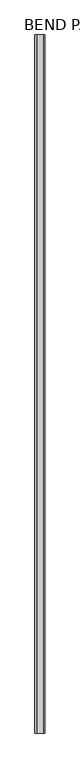
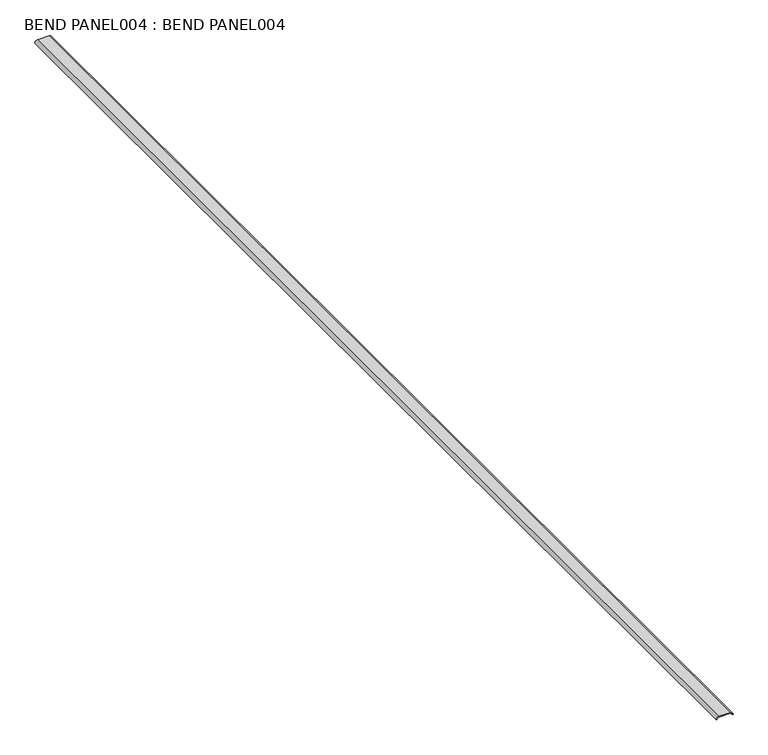
"""IFC4 building model written with IfcOpenShell, lengths in millimetres: proxy geometry, BEND PANEL004 : BEND PANEL004."""

import ifcopenshell
import ifcopenshell.guid

model = None  # the IFC model being written
_history = None  # IfcOwnerHistory: only IFC2X3 demands one
_inside = {}  # id of a spatial element -> (the spatial element, [elements in it])
_under = {}  # id of a project, library or spatial element -> (it, [spatial elements below it])
_declared = {}  # id of a project -> (the project, [libraries it declares])
_typed = {}  # id of a type object -> (the type object, [elements of that type])
_made_of = {}  # id of a material, layer set ... -> (it, [elements and type objects made of it])


def new_model(schema):
    """Start an empty IFC model of exactly this schema.

    Asked for "IFC4X3", IfcOpenShell would pick the latest addendum, in which some entities
    have other attributes; the version numbers below select the first issue.
    IFC2X3 requires an IfcOwnerHistory on every rooted entity: one is made here for all.
    """
    global model, _history
    if schema == "IFC4X3":
        model = ifcopenshell.file(schema_version=(4, 3, 0, 0))
    else:
        model = ifcopenshell.file(schema=schema)
    _inside.clear()
    _under.clear()
    _declared.clear()
    _typed.clear()
    _made_of.clear()
    _history = None
    if model.schema == "IFC2X3":
        org = make("IfcOrganization", Name="unknown")
        user = make(
            "IfcPersonAndOrganization",
            ThePerson=make("IfcPerson", FamilyName="unknown"),
            TheOrganization=org,
        )
        app = make(
            "IfcApplication",
            ApplicationDeveloper=org,
            Version="unknown",
            ApplicationFullName="unknown",
            ApplicationIdentifier="unknown",
        )
        _history = make(
            "IfcOwnerHistory",
            OwningUser=user,
            OwningApplication=app,
            ChangeAction="ADDED",
            CreationDate=0,
        )
    return model


def make(cls, **values):
    """One entity of the class cls with the attributes given. An attribute that is None is left unset."""
    return model.create_entity(
        cls, **{name: value for name, value in values.items() if value is not None}
    )


def rooted(cls, **values):
    """An entity with a GlobalId (a new one), such as an element, a storey or a relation."""
    return make(cls, GlobalId=ifcopenshell.guid.new(), OwnerHistory=_history, **values)


def si_unit(unit_type, name, prefix=None):
    """IfcSIUnit, for example si_unit("LENGTHUNIT", "METRE", prefix="MILLI")."""
    return make("IfcSIUnit", UnitType=unit_type, Prefix=prefix, Name=name)


def assignment(units):
    """IfcUnitAssignment: the units of a project."""
    return None if units is None else make("IfcUnitAssignment", Units=units)


def point(xyz):
    """IfcCartesianPoint."""
    return None if xyz is None else make("IfcCartesianPoint", Coordinates=xyz)


def direction(xyz):
    """IfcDirection."""
    return None if xyz is None else make("IfcDirection", DirectionRatios=xyz)


def frame(location, z_axis=None, x_axis=None):
    """IfcAxis2Placement3D, a coordinate frame: its origin and axes. An axis left out is left unset."""
    return make(
        "IfcAxis2Placement3D",
        Location=point(location),
        Axis=direction(z_axis),
        RefDirection=direction(x_axis),
    )


def frame_2d(location, x_axis=None):
    """IfcAxis2Placement2D, a coordinate frame in the plane: its origin and x axis."""
    return make(
        "IfcAxis2Placement2D", Location=point(location), RefDirection=direction(x_axis)
    )


def origin():
    """The frame at (0, 0, 0) with its axes left unset."""
    return frame((0.0, 0.0, 0.0))


def place(relative_to, where):
    """IfcLocalPlacement: puts the frame where relative to a parent placement (None: the world)."""
    return make(
        "IfcLocalPlacement", PlacementRelTo=relative_to, RelativePlacement=where
    )


def context(
    kind, dimensions, precision=None, world=None, true_north=None, identifier=None
):
    """IfcGeometricRepresentationContext, for example the 3D "Model" context."""
    return make(
        "IfcGeometricRepresentationContext",
        ContextIdentifier=identifier,
        ContextType=kind,
        CoordinateSpaceDimension=dimensions,
        Precision=precision,
        WorldCoordinateSystem=world,
        TrueNorth=true_north,
    )


def project(units=None, contexts=None):
    """IfcProject with its units and contexts."""
    return rooted(
        "IfcProject",
        Name="project",
        RepresentationContexts=contexts,
        UnitsInContext=assignment(units),
    )


def spatial(cls, under=None, at=None, **own):
    """A site, building, storey or space (cls), placed at a placement, below another one or the project."""
    s = rooted(cls, ObjectPlacement=at, **own)
    if under is not None:
        _under.setdefault(under.id(), (under, []))[1].append(s)
    return s


def polyline(points):
    """IfcPolyline through the points."""
    return make("IfcPolyline", Points=[point(p) for p in points])


def circle_curve(where, radius):
    """IfcCircle in the frame where."""
    return make("IfcCircle", Position=where, Radius=radius)


def trimmed(basis, trim1, trim2, sense, master):
    """IfcTrimmedCurve: the piece of a basis curve between two trims."""
    return make(
        "IfcTrimmedCurve",
        BasisCurve=basis,
        Trim1=trim1,
        Trim2=trim2,
        SenseAgreement=sense,
        MasterRepresentation=master,
    )


def segment(curve, same_sense, transition):
    """IfcCompositeCurveSegment."""
    return make(
        "IfcCompositeCurveSegment",
        Transition=transition,
        SameSense=same_sense,
        ParentCurve=curve,
    )


def composite_curve(segments, self_intersect=None):
    """IfcCompositeCurve: segments joined end to end."""
    return make("IfcCompositeCurve", Segments=segments, SelfIntersect=self_intersect)


def outline(outer, holes=None, kind="AREA"):
    """IfcArbitraryClosedProfileDef: a profile drawn as a closed curve; with holes, ...WithVoids."""
    if holes is None:
        return make("IfcArbitraryClosedProfileDef", ProfileType=kind, OuterCurve=outer)
    return make(
        "IfcArbitraryProfileDefWithVoids",
        ProfileType=kind,
        OuterCurve=outer,
        InnerCurves=holes,
    )


def extrude(swept, where, along, depth):
    """IfcExtrudedAreaSolid: the profile swept, set in the frame where, extruded along a direction by depth."""
    return make(
        "IfcExtrudedAreaSolid",
        SweptArea=swept,
        Position=where,
        ExtrudedDirection=direction(along),
        Depth=depth,
    )


def shape(context_of_items, identifier, shape_type, items):
    """IfcShapeRepresentation: the items that make up one representation, for example the "Body"."""
    return make(
        "IfcShapeRepresentation",
        ContextOfItems=context_of_items,
        RepresentationIdentifier=identifier,
        RepresentationType=shape_type,
        Items=items,
    )


def source(mapping_origin, context_of_items, identifier, shape_type, items):
    """IfcRepresentationMap: a shape defined once, which mapped items show again and again."""
    return make(
        "IfcRepresentationMap",
        MappingOrigin=mapping_origin,
        MappedRepresentation=shape(context_of_items, identifier, shape_type, items),
    )


def transform(
    local_origin,
    x_axis=None,
    y_axis=None,
    z_axis=None,
    scale=None,
    scale2=None,
    scale3=None,
    uniform=True,
):
    """IfcCartesianTransformationOperator3D, or its non-uniform kind. x_axis, y_axis, z_axis: its Axis1, 2, 3."""
    if uniform:
        return make(
            "IfcCartesianTransformationOperator3D",
            Axis1=direction(x_axis),
            Axis2=direction(y_axis),
            LocalOrigin=point(local_origin),
            Scale=scale,
            Axis3=direction(z_axis),
        )
    return make(
        "IfcCartesianTransformationOperator3DnonUniform",
        Axis1=direction(x_axis),
        Axis2=direction(y_axis),
        LocalOrigin=point(local_origin),
        Scale=scale,
        Axis3=direction(z_axis),
        Scale2=scale2,
        Scale3=scale3,
    )


def mapped(mapping_source, mapping_target):
    """IfcMappedItem: shows the shape of a source again, moved by a transform."""
    return make(
        "IfcMappedItem", MappingSource=mapping_source, MappingTarget=mapping_target
    )


def made_of(thing, what):
    """Note that an element or type object is made of a material, layer set ...; save() writes the relation."""
    if what is not None:
        _made_of.setdefault(what.id(), (what, []))[1].append(thing)
    return thing


def element(
    cls,
    number,
    at=None,
    inside=None,
    cuts=None,
    type_object=None,
    material=None,
    context=None,
    identifier="Body",
    shape_type=None,
    held_by="IfcProductDefinitionShape",
    body=None,
    shapes=None,
    **own,
):
    """One element of the class cls, such as IfcWall. Its Tag is "e" and its number.

    at: its placement. inside: the storey or other place that contains it. cuts: it is an
    opening in that element (IfcRelVoidsElement). A single representation is given by context,
    identifier, shape_type and body (its items); several are given by shapes. held_by: the class
    of the entity that holds the representations. save() writes the other relations.
    """
    e = rooted(cls, Tag="e%d" % number, ObjectPlacement=at, **own)
    if body is not None:
        shapes = [shape(context, identifier, shape_type, body)]
    if shapes is not None:
        e.Representation = make(held_by, Representations=shapes)
    if inside is not None:
        _inside.setdefault(inside.id(), (inside, []))[1].append(e)
    if cuts is not None:
        rooted(
            "IfcRelVoidsElement", RelatingBuildingElement=cuts, RelatedOpeningElement=e
        )
    if type_object is not None:
        _typed.setdefault(type_object.id(), (type_object, []))[1].append(e)
    return made_of(e, material)


def aggregate(whole, parts):
    """IfcRelAggregates: a whole, such as a stair, and the parts it consists of."""
    return rooted("IfcRelAggregates", RelatingObject=whole, RelatedObjects=parts)


def save(model, path):
    """Write the relations noted so far, then the file.

    IfcRelAggregates (storeys below a building ...), IfcRelContainedInSpatialStructure (elements
    in a storey), IfcRelDefinesByType, IfcRelAssociatesMaterial and IfcRelDeclares: one each for
    every whole, place, type object, material and project.
    """
    for whole, parts in _under.values():
        aggregate(whole, parts)
    for where, things in _inside.values():
        rooted(
            "IfcRelContainedInSpatialStructure",
            RelatedElements=things,
            RelatingStructure=where,
        )
    for kind, things in _typed.values():
        rooted("IfcRelDefinesByType", RelatedObjects=things, RelatingType=kind)
    for what, things in _made_of.values():
        rooted("IfcRelAssociatesMaterial", RelatedObjects=things, RelatingMaterial=what)
    for by, libraries in _declared.values():
        rooted("IfcRelDeclares", RelatingContext=by, RelatedDefinitions=libraries)
    model.write(path)


def bend_panel004_bend_panel004_15d214a6(model_context):
    return source(origin(), model_context, "Body", "SweptSolid", [
        extrude(outline(composite_curve([segment(polyline([(42576.61192, 5858.4004637), (42576.61192, 5859.5910887)]), True, "CONTINUOUS"), segment(trimmed(circle_curve(frame_2d((42576.6119199, 5862.9993652)), 3.4082764), [point((42576.61192, 5859.5910887))], [point((42580.0201795, 5863.0100787))], True, "CARTESIAN"), True, "CONTINUOUS"), segment(polyline([(42580.0201795, 5863.0100787), (42580.0201963, 5882.3645691)]), True, "CONTINUOUS"), segment(trimmed(circle_curve(frame_2d((42576.6119199, 5882.3645721)), 3.4082764), [point((42580.0201963, 5882.3645691))], [point((42576.61192, 5885.7728485))], True, "CARTESIAN"), True, "CONTINUOUS"), segment(polyline([(42576.61192, 5885.7728485), (42576.61192, 5886.9634735)]), True, "CONTINUOUS"), segment(trimmed(circle_curve(frame_2d((42576.6119199, 5882.3645721)), 4.5989014), [point((42576.61192, 5886.9634735))], [point((42581.2108213, 5882.364568))], False, "CARTESIAN"), True, "CONTINUOUS"), segment(polyline([(42581.2108213, 5882.364568), (42581.2108045, 5863.0118181)]), True, "CONTINUOUS"), segment(trimmed(circle_curve(frame_2d((42576.6119199, 5862.9993652)), 4.5989014), [point((42581.2108045, 5863.0118181))], [point((42576.61192, 5858.4004637))], False, "CARTESIAN"), True, "CONTINUOUS")], self_intersect=False)), frame((0.0, -1052.8906574, 0.0), z_axis=(0.0, 1.0, 0.0), x_axis=(0.0, 0.0, 1.0)), (0.0, 0.0, 1.0), 1999.85),
    ])


if __name__ == "__main__":
    model = new_model("IFC4")
    model_context = context("Model", 3, world=origin())
    ifc_project = project(units=[si_unit("LENGTHUNIT", "METRE", prefix="MILLI")], contexts=[model_context])
    site = spatial("IfcSite", under=ifc_project)
    building = spatial("IfcBuilding", under=site)
    placement = place(None, origin())
    bend_panel004_bend_panel004_shape = bend_panel004_bend_panel004_15d214a6(model_context)
    element("IfcBuildingElementProxy", 1, Name="BEND PANEL004 : BEND PANEL004", ObjectType="BEND PANEL004 : BEND PANEL004", at=placement, inside=building, context=model_context, shape_type="MappedRepresentation", body=[
        mapped(bend_panel004_bend_panel004_shape, transform((0.0, 0.0, 0.0), x_axis=(1.0, 0.0, 0.0), y_axis=(0.0, 1.0, 0.0), z_axis=(0.0, 0.0, 1.0))),
    ])
    save(model, "model.ifc")

# Revit data of these elements
# Type "BEND PANEL004 : BEND PANEL004"
#   NameOverride = "BEND PANEL004"
# Element 1 (IfcBuildingElementProxy, "BEND PANEL004 : BEND PANEL004")
#   Materials on its faces: "METAL PROFILE"
# Materials
#   "METAL PROFILE": class "Unassigned", colour RGB 128 128 128, transparency 0
